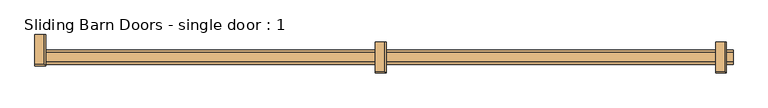
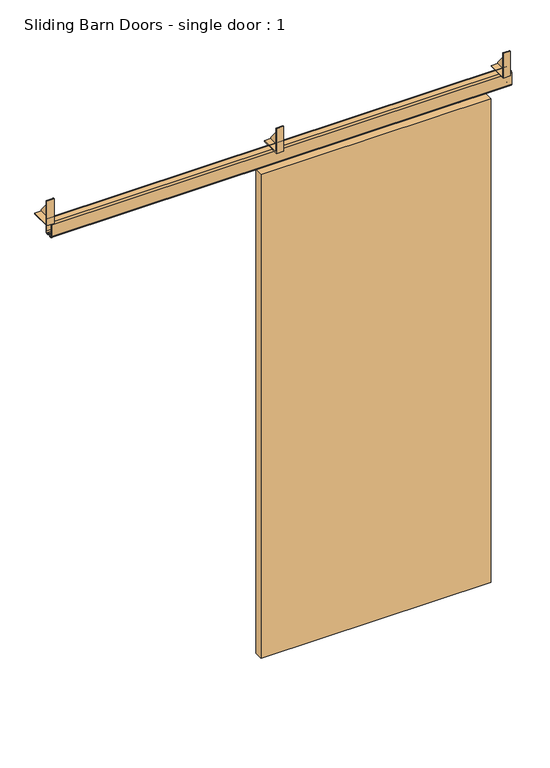
"""IFC4 building model written with IfcOpenShell, lengths in millimetres: door geometry, Sliding Barn Doors - single door : 1."""

from ifc_helpers import new_model, si_unit, point, frame, frame_2d, origin, place, context, project, spatial, polyline, circle_curve, trimmed, segment, composite_curve, outline, extrude, source, transform, mapped, element, save


def sliding_barn_doors_single_door_1_980e15fc(model_context):
    return source(origin(), model_context, "Body", "SweptSolid", [
        extrude(outline(polyline([(158.75, 2152.65), (158.75, 2146.3), (79.375, 2146.3), (79.375, 2247.773), (158.75, 2152.65)])), frame((-1385.9371094, 0.0, 0.0), z_axis=(1.0, 0.0, 0.0), x_axis=(0.0, 1.0, 0.0)), (0.0, 0.0, 1.0), 3.175),
        extrude(outline(polyline([(76.2, 2143.125), (76.2, 2247.773), (79.375, 2247.773), (79.375, 2146.3), (158.75, 2146.3), (158.75, 2143.125), (76.2, 2143.125)])), frame((-1411.2378906, 0.0, 0.0), z_axis=(1.0, 0.0, 0.0), x_axis=(0.0, 1.0, 0.0)), (0.0, 0.0, 1.0), 28.4757812),
        extrude(outline(polyline([(139.7, 2152.65), (139.7, 2146.3), (60.325, 2146.3), (60.325, 2247.773), (139.7, 2152.65)])), frame((-484.2371094, 0.0, 0.0), z_axis=(1.0, 0.0, 0.0), x_axis=(0.0, 1.0, 0.0)), (0.0, 0.0, 1.0), 3.175),
        extrude(outline(polyline([(57.15, 2143.125), (57.15, 2247.773), (60.325, 2247.773), (60.325, 2146.3), (139.7, 2146.3), (139.7, 2143.125), (57.15, 2143.125)])), frame((-509.5378906, 0.0, 0.0), z_axis=(1.0, 0.0, 0.0), x_axis=(0.0, 1.0, 0.0)), (0.0, 0.0, 1.0), 28.4757813),
        extrude(outline(polyline([(139.7, 2152.65), (139.7, 2146.3), (60.325, 2146.3), (60.325, 2247.773), (139.7, 2152.65)])), frame((417.4628906, 0.0, 0.0), z_axis=(1.0, 0.0, 0.0), x_axis=(0.0, 1.0, 0.0)), (0.0, 0.0, 1.0), 3.175),
        extrude(outline(polyline([(57.15, 2143.125), (57.15, 2247.773), (60.325, 2247.773), (60.325, 2146.3), (139.7, 2146.3), (139.7, 2143.125), (57.15, 2143.125)])), frame((392.1621094, 0.0, 0.0), z_axis=(1.0, 0.0, 0.0), x_axis=(0.0, 1.0, 0.0)), (0.0, 0.0, 1.0), 28.4757813),
        extrude(outline(polyline([(-457.454, 117.475), (-406.146, 117.475), (-406.146, 114.3), (-457.454, 114.3), (-457.454, 117.475)])), frame((0.0, 0.0, 1889.252), z_axis=(0.0, 0.0, 1.0), x_axis=(1.0, 0.0, 0.0)), (0.0, 0.0, 1.0), 168.148),
        extrude(outline(polyline([(202.946, 117.475), (254.254, 117.475), (254.254, 114.3), (202.946, 114.3), (202.946, 117.475)])), frame((0.0, 0.0, 1889.252), z_axis=(0.0, 0.0, 1.0), x_axis=(1.0, 0.0, 0.0)), (0.0, 0.0, 1.0), 168.148),
        extrude(outline(polyline([(-558.8, 114.3), (355.6, 114.3), (355.6, 79.375), (-558.8, 79.375), (-558.8, 114.3)])), frame((0.0, 0.0, 25.4), z_axis=(0.0, 0.0, 1.0), x_axis=(1.0, 0.0, 0.0)), (0.0, 0.0, 1.0), 2032.0),
        extrude(outline(composite_curve([segment(polyline([(85.725, 2143.125), (111.252, 2143.125)]), True, "CONTINUOUS"), segment(trimmed(circle_curve(frame_2d((111.252, 2136.775)), 6.35), [point((111.252, 2143.125))], [point((117.602, 2136.775))], False, "CARTESIAN"), True, "CONTINUOUS"), segment(polyline([(117.602, 2136.775), (117.602, 2088.515)]), True, "CONTINUOUS"), segment(trimmed(circle_curve(frame_2d((111.252, 2088.515)), 6.35), [point((117.602, 2088.515))], [point((111.252, 2082.165))], False, "CARTESIAN"), True, "CONTINUOUS"), segment(polyline([(111.252, 2082.165), (105.8433147, 2082.165)]), True, "CONTINUOUS"), segment(trimmed(circle_curve(frame_2d((105.8433147, 2083.7525)), 1.5875), [point((105.8433147, 2082.165))], [point((104.2849816, 2083.4495907))], False, "CARTESIAN"), True, "CONTINUOUS"), segment(polyline([(104.2849816, 2083.4495907), (102.8594659, 2090.7832331), (104.3756029, 2090.7832331), (105.7615251, 2083.6532812), (111.252, 2083.6532812)]), True, "CONTINUOUS"), segment(trimmed(circle_curve(frame_2d((111.252, 2088.515)), 4.8617187), [point((111.252, 2083.6532812))], [point((116.1137188, 2088.515))], True, "CARTESIAN"), True, "CONTINUOUS"), segment(polyline([(116.1137188, 2088.515), (116.1137188, 2136.775)]), True, "CONTINUOUS"), segment(trimmed(circle_curve(frame_2d((111.252, 2136.775)), 4.8617187), [point((116.1137188, 2136.775))], [point((111.252, 2141.6367187))], True, "CARTESIAN"), True, "CONTINUOUS"), segment(polyline([(111.252, 2141.6367187), (85.725, 2141.6367187)]), True, "CONTINUOUS"), segment(trimmed(circle_curve(frame_2d((85.725, 2136.775)), 4.8617187), [point((85.725, 2141.6367187))], [point((80.8632813, 2136.775))], True, "CARTESIAN"), True, "CONTINUOUS"), segment(polyline([(80.8632813, 2136.775), (80.8632813, 2088.515)]), True, "CONTINUOUS"), segment(trimmed(circle_curve(frame_2d((85.725, 2088.515)), 4.8617187), [point((80.8632813, 2088.515))], [point((85.725, 2083.6532812))], True, "CARTESIAN"), True, "CONTINUOUS"), segment(polyline([(85.725, 2083.6532812), (91.2154749, 2083.6532812), (92.6013971, 2090.7832331), (94.1175341, 2090.7832331), (92.6920184, 2083.4495907)]), True, "CONTINUOUS"), segment(trimmed(circle_curve(frame_2d((91.1336853, 2083.7525)), 1.5875), [point((92.6920184, 2083.4495907))], [point((91.1336853, 2082.165))], False, "CARTESIAN"), True, "CONTINUOUS"), segment(polyline([(91.1336853, 2082.165), (85.725, 2082.165)]), True, "CONTINUOUS"), segment(trimmed(circle_curve(frame_2d((85.725, 2088.515)), 6.35), [point((85.725, 2082.165))], [point((79.375, 2088.515))], False, "CARTESIAN"), True, "CONTINUOUS"), segment(polyline([(79.375, 2088.515), (79.375, 2136.775)]), True, "CONTINUOUS"), segment(trimmed(circle_curve(frame_2d((85.725, 2136.775)), 6.35), [point((79.375, 2136.775))], [point((85.725, 2143.125))], False, "CARTESIAN"), True, "CONTINUOUS")], self_intersect=False)), frame((-1390.65, 0.0, 0.0), z_axis=(1.0, 0.0, 0.0), x_axis=(0.0, 1.0, 0.0)), (0.0, 0.0, 1.0), 1828.8),
    ])


if __name__ == "__main__":
    model = new_model("IFC4")
    model_context = context("Model", 3, world=origin())
    ifc_project = project(units=[si_unit("LENGTHUNIT", "METRE", prefix="MILLI")], contexts=[model_context])
    site = spatial("IfcSite", under=ifc_project)
    building = spatial("IfcBuilding", under=site)
    placement = place(None, origin())
    sliding_barn_doors_single_door_1_shape = sliding_barn_doors_single_door_1_980e15fc(model_context)
    element("IfcDoor", 1, ObjectType="Sliding Barn Doors - single door : 1", at=placement, inside=building, context=model_context, shape_type="MappedRepresentation", body=[
        mapped(sliding_barn_doors_single_door_1_shape, transform((0.0, 0.0, 0.0), x_axis=(1.0, 0.0, 0.0), y_axis=(0.0, 1.0, 0.0), z_axis=(0.0, 0.0, 1.0))),
    ])
    save(model, "model.ifc")

# Revit data of these elements
# Type "Sliding Barn Doors - single door : 1"
#   Type Mark = "61"
#   OD_DS_Door_Material = "T.B.D."
#   OD_DS_Door_Type = "SLIDER"
#   OD_DS_Lockset = "-"
#   Analytic Construction = "<None>"
#   rail_overlap_left = 0' - 5 1/4"
#   rail_length = 6' - 0"
#   overlap_left = 0' - 2"
#   overlap = 0' - 0"
#   bracket_right = 3' - 7"
#   bracket_left = 0' - 4"
#   Thickness = 0' - 1 3/8"
#   Panel Width = 3' - 0"
#   Panel Height = 6' - 8"
#   Gap 2 = 0' - 0 1/2"
#   Gap 1 = 0' - 0 7/8"
#   Frame Projection Ext. = 0' - 1"
#   Frame Projection Int. = 0' - 1"
#   Frame Width = 0' - 3"
#   Height = 6' - 4"
#   Width = 2' - 0"
#   Bracket_offset = 0' - 5"
#   Door_4 = no
#   Door_3 = no
#   Hardware Material = Metal - Aluminum
#   Door Material = Closet_1
#   Function = (empty or 0)
#   Wall Closure = (empty or 0)
# Element 1 (IfcDoor, "Sliding Barn Doors - single door : 1")
#   Materials on its faces: "Metal - Aluminum", "Closet_1"
# Materials
#   "Metal - Aluminum": class "Metal", colour RGB 247 247 247, transparency 0
#   "Closet_1": class "Paint", colour RGB 200 194 183, transparency 0, Cost = 0
